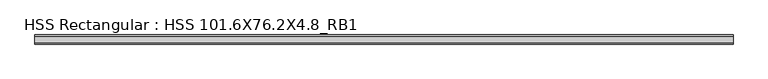
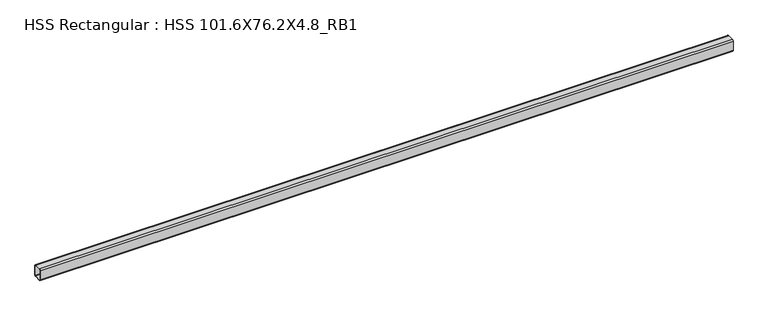
"""IFC4 building model written with IfcOpenShell, lengths in millimetres: beam geometry, HSS Rectangular : HSS 101.6X76.2X4.8_RB1."""

import ifcopenshell
import ifcopenshell.guid

model = None  # the IFC model being written
_history = None  # IfcOwnerHistory: only IFC2X3 demands one
_inside = {}  # id of a spatial element -> (the spatial element, [elements in it])
_under = {}  # id of a project, library or spatial element -> (it, [spatial elements below it])
_declared = {}  # id of a project -> (the project, [libraries it declares])
_typed = {}  # id of a type object -> (the type object, [elements of that type])
_made_of = {}  # id of a material, layer set ... -> (it, [elements and type objects made of it])


def new_model(schema):
    """Start an empty IFC model of exactly this schema.

    Asked for "IFC4X3", IfcOpenShell would pick the latest addendum, in which some entities
    have other attributes; the version numbers below select the first issue.
    IFC2X3 requires an IfcOwnerHistory on every rooted entity: one is made here for all.
    """
    global model, _history
    if schema == "IFC4X3":
        model = ifcopenshell.file(schema_version=(4, 3, 0, 0))
    else:
        model = ifcopenshell.file(schema=schema)
    _inside.clear()
    _under.clear()
    _declared.clear()
    _typed.clear()
    _made_of.clear()
    _history = None
    if model.schema == "IFC2X3":
        org = make("IfcOrganization", Name="unknown")
        user = make(
            "IfcPersonAndOrganization",
            ThePerson=make("IfcPerson", FamilyName="unknown"),
            TheOrganization=org,
        )
        app = make(
            "IfcApplication",
            ApplicationDeveloper=org,
            Version="unknown",
            ApplicationFullName="unknown",
            ApplicationIdentifier="unknown",
        )
        _history = make(
            "IfcOwnerHistory",
            OwningUser=user,
            OwningApplication=app,
            ChangeAction="ADDED",
            CreationDate=0,
        )
    return model


def make(cls, **values):
    """One entity of the class cls with the attributes given. An attribute that is None is left unset."""
    return model.create_entity(
        cls, **{name: value for name, value in values.items() if value is not None}
    )


def rooted(cls, **values):
    """An entity with a GlobalId (a new one), such as an element, a storey or a relation."""
    return make(cls, GlobalId=ifcopenshell.guid.new(), OwnerHistory=_history, **values)


def si_unit(unit_type, name, prefix=None):
    """IfcSIUnit, for example si_unit("LENGTHUNIT", "METRE", prefix="MILLI")."""
    return make("IfcSIUnit", UnitType=unit_type, Prefix=prefix, Name=name)


def assignment(units):
    """IfcUnitAssignment: the units of a project."""
    return None if units is None else make("IfcUnitAssignment", Units=units)


def point(xyz):
    """IfcCartesianPoint."""
    return None if xyz is None else make("IfcCartesianPoint", Coordinates=xyz)


def direction(xyz):
    """IfcDirection."""
    return None if xyz is None else make("IfcDirection", DirectionRatios=xyz)


def frame(location, z_axis=None, x_axis=None):
    """IfcAxis2Placement3D, a coordinate frame: its origin and axes. An axis left out is left unset."""
    return make(
        "IfcAxis2Placement3D",
        Location=point(location),
        Axis=direction(z_axis),
        RefDirection=direction(x_axis),
    )


def frame_2d(location, x_axis=None):
    """IfcAxis2Placement2D, a coordinate frame in the plane: its origin and x axis."""
    return make(
        "IfcAxis2Placement2D", Location=point(location), RefDirection=direction(x_axis)
    )


def origin():
    """The frame at (0, 0, 0) with its axes left unset."""
    return frame((0.0, 0.0, 0.0))


def place(relative_to, where):
    """IfcLocalPlacement: puts the frame where relative to a parent placement (None: the world)."""
    return make(
        "IfcLocalPlacement", PlacementRelTo=relative_to, RelativePlacement=where
    )


def context(
    kind, dimensions, precision=None, world=None, true_north=None, identifier=None
):
    """IfcGeometricRepresentationContext, for example the 3D "Model" context."""
    return make(
        "IfcGeometricRepresentationContext",
        ContextIdentifier=identifier,
        ContextType=kind,
        CoordinateSpaceDimension=dimensions,
        Precision=precision,
        WorldCoordinateSystem=world,
        TrueNorth=true_north,
    )


def project(units=None, contexts=None):
    """IfcProject with its units and contexts."""
    return rooted(
        "IfcProject",
        Name="project",
        RepresentationContexts=contexts,
        UnitsInContext=assignment(units),
    )


def spatial(cls, under=None, at=None, **own):
    """A site, building, storey or space (cls), placed at a placement, below another one or the project."""
    s = rooted(cls, ObjectPlacement=at, **own)
    if under is not None:
        _under.setdefault(under.id(), (under, []))[1].append(s)
    return s


def polyline(points):
    """IfcPolyline through the points."""
    return make("IfcPolyline", Points=[point(p) for p in points])


def circle_curve(where, radius):
    """IfcCircle in the frame where."""
    return make("IfcCircle", Position=where, Radius=radius)


def trimmed(basis, trim1, trim2, sense, master):
    """IfcTrimmedCurve: the piece of a basis curve between two trims."""
    return make(
        "IfcTrimmedCurve",
        BasisCurve=basis,
        Trim1=trim1,
        Trim2=trim2,
        SenseAgreement=sense,
        MasterRepresentation=master,
    )


def segment(curve, same_sense, transition):
    """IfcCompositeCurveSegment."""
    return make(
        "IfcCompositeCurveSegment",
        Transition=transition,
        SameSense=same_sense,
        ParentCurve=curve,
    )


def composite_curve(segments, self_intersect=None):
    """IfcCompositeCurve: segments joined end to end."""
    return make("IfcCompositeCurve", Segments=segments, SelfIntersect=self_intersect)


def outline(outer, holes=None, kind="AREA"):
    """IfcArbitraryClosedProfileDef: a profile drawn as a closed curve; with holes, ...WithVoids."""
    if holes is None:
        return make("IfcArbitraryClosedProfileDef", ProfileType=kind, OuterCurve=outer)
    return make(
        "IfcArbitraryProfileDefWithVoids",
        ProfileType=kind,
        OuterCurve=outer,
        InnerCurves=holes,
    )


def extrude(swept, where, along, depth):
    """IfcExtrudedAreaSolid: the profile swept, set in the frame where, extruded along a direction by depth."""
    return make(
        "IfcExtrudedAreaSolid",
        SweptArea=swept,
        Position=where,
        ExtrudedDirection=direction(along),
        Depth=depth,
    )


def shape(context_of_items, identifier, shape_type, items):
    """IfcShapeRepresentation: the items that make up one representation, for example the "Body"."""
    return make(
        "IfcShapeRepresentation",
        ContextOfItems=context_of_items,
        RepresentationIdentifier=identifier,
        RepresentationType=shape_type,
        Items=items,
    )


def source(mapping_origin, context_of_items, identifier, shape_type, items):
    """IfcRepresentationMap: a shape defined once, which mapped items show again and again."""
    return make(
        "IfcRepresentationMap",
        MappingOrigin=mapping_origin,
        MappedRepresentation=shape(context_of_items, identifier, shape_type, items),
    )


def transform(
    local_origin,
    x_axis=None,
    y_axis=None,
    z_axis=None,
    scale=None,
    scale2=None,
    scale3=None,
    uniform=True,
):
    """IfcCartesianTransformationOperator3D, or its non-uniform kind. x_axis, y_axis, z_axis: its Axis1, 2, 3."""
    if uniform:
        return make(
            "IfcCartesianTransformationOperator3D",
            Axis1=direction(x_axis),
            Axis2=direction(y_axis),
            LocalOrigin=point(local_origin),
            Scale=scale,
            Axis3=direction(z_axis),
        )
    return make(
        "IfcCartesianTransformationOperator3DnonUniform",
        Axis1=direction(x_axis),
        Axis2=direction(y_axis),
        LocalOrigin=point(local_origin),
        Scale=scale,
        Axis3=direction(z_axis),
        Scale2=scale2,
        Scale3=scale3,
    )


def mapped(mapping_source, mapping_target):
    """IfcMappedItem: shows the shape of a source again, moved by a transform."""
    return make(
        "IfcMappedItem", MappingSource=mapping_source, MappingTarget=mapping_target
    )


def made_of(thing, what):
    """Note that an element or type object is made of a material, layer set ...; save() writes the relation."""
    if what is not None:
        _made_of.setdefault(what.id(), (what, []))[1].append(thing)
    return thing


def element(
    cls,
    number,
    at=None,
    inside=None,
    cuts=None,
    type_object=None,
    material=None,
    context=None,
    identifier="Body",
    shape_type=None,
    held_by="IfcProductDefinitionShape",
    body=None,
    shapes=None,
    **own,
):
    """One element of the class cls, such as IfcWall. Its Tag is "e" and its number.

    at: its placement. inside: the storey or other place that contains it. cuts: it is an
    opening in that element (IfcRelVoidsElement). A single representation is given by context,
    identifier, shape_type and body (its items); several are given by shapes. held_by: the class
    of the entity that holds the representations. save() writes the other relations.
    """
    e = rooted(cls, Tag="e%d" % number, ObjectPlacement=at, **own)
    if body is not None:
        shapes = [shape(context, identifier, shape_type, body)]
    if shapes is not None:
        e.Representation = make(held_by, Representations=shapes)
    if inside is not None:
        _inside.setdefault(inside.id(), (inside, []))[1].append(e)
    if cuts is not None:
        rooted(
            "IfcRelVoidsElement", RelatingBuildingElement=cuts, RelatedOpeningElement=e
        )
    if type_object is not None:
        _typed.setdefault(type_object.id(), (type_object, []))[1].append(e)
    return made_of(e, material)


def aggregate(whole, parts):
    """IfcRelAggregates: a whole, such as a stair, and the parts it consists of."""
    return rooted("IfcRelAggregates", RelatingObject=whole, RelatedObjects=parts)


def save(model, path):
    """Write the relations noted so far, then the file.

    IfcRelAggregates (storeys below a building ...), IfcRelContainedInSpatialStructure (elements
    in a storey), IfcRelDefinesByType, IfcRelAssociatesMaterial and IfcRelDeclares: one each for
    every whole, place, type object, material and project.
    """
    for whole, parts in _under.values():
        aggregate(whole, parts)
    for where, things in _inside.values():
        rooted(
            "IfcRelContainedInSpatialStructure",
            RelatedElements=things,
            RelatingStructure=where,
        )
    for kind, things in _typed.values():
        rooted("IfcRelDefinesByType", RelatedObjects=things, RelatingType=kind)
    for what, things in _made_of.values():
        rooted("IfcRelAssociatesMaterial", RelatedObjects=things, RelatingMaterial=what)
    for by, libraries in _declared.values():
        rooted("IfcRelDeclares", RelatingContext=by, RelatedDefinitions=libraries)
    model.write(path)


def hss_rectangular_hss_101_6x76_2x4_8_rb1_d55246ad(model_context):
    return source(origin(), model_context, "Body", "SweptSolid", [
        extrude(outline(composite_curve([segment(polyline([(38.1, 41.275), (38.1, -41.275)]), True, "CONTINUOUS"), segment(trimmed(circle_curve(frame_2d((28.575, -41.275)), 9.525), [point((38.1, -41.275))], [point((28.575, -50.8))], False, "CARTESIAN"), True, "CONTINUOUS"), segment(polyline([(28.575, -50.8), (-28.575, -50.8)]), True, "CONTINUOUS"), segment(trimmed(circle_curve(frame_2d((-28.575, -41.275)), 9.525), [point((-28.575, -50.8))], [point((-38.1, -41.275))], False, "CARTESIAN"), True, "CONTINUOUS"), segment(polyline([(-38.1, -41.275), (-38.1, 41.275)]), True, "CONTINUOUS"), segment(trimmed(circle_curve(frame_2d((-28.575, 41.275)), 9.525), [point((-38.1, 41.275))], [point((-28.575, 50.8))], False, "CARTESIAN"), True, "CONTINUOUS"), segment(polyline([(-28.575, 50.8), (28.575, 50.8)]), True, "CONTINUOUS"), segment(trimmed(circle_curve(frame_2d((28.575, 41.275)), 9.525), [point((28.575, 50.8))], [point((38.1, 41.275))], False, "CARTESIAN"), True, "CONTINUOUS")], self_intersect=False), holes=[composite_curve([segment(trimmed(circle_curve(frame_2d((-28.575, 41.275)), 4.7625), [point((-28.575, 46.0375))], [point((-33.3375, 41.275))], True, "CARTESIAN"), True, "CONTINUOUS"), segment(polyline([(-33.3375, 41.275), (-33.3375, -41.275)]), True, "CONTINUOUS"), segment(trimmed(circle_curve(frame_2d((-28.575, -41.275)), 4.7625), [point((-33.3375, -41.275))], [point((-28.575, -46.0375))], True, "CARTESIAN"), True, "CONTINUOUS"), segment(polyline([(-28.575, -46.0375), (28.575, -46.0375)]), True, "CONTINUOUS"), segment(trimmed(circle_curve(frame_2d((28.575, -41.275)), 4.7625), [point((28.575, -46.0375))], [point((33.3375, -41.275))], True, "CARTESIAN"), True, "CONTINUOUS"), segment(polyline([(33.3375, -41.275), (33.3375, 41.275)]), True, "CONTINUOUS"), segment(trimmed(circle_curve(frame_2d((28.575, 41.275)), 4.7625), [point((33.3375, 41.275))], [point((28.575, 46.0375))], True, "CARTESIAN"), True, "CONTINUOUS"), segment(polyline([(28.575, 46.0375), (-28.575, 46.0375)]), True, "CONTINUOUS")], self_intersect=False)]), frame((-7467.2727012, 0.0, 0.0), z_axis=(1.0, 0.0, 0.0), x_axis=(0.0, 1.0, 0.0)), (0.0, 0.0, 1.0), 5840.0992104),
    ])


if __name__ == "__main__":
    model = new_model("IFC4")
    model_context = context("Model", 3, world=origin())
    ifc_project = project(units=[si_unit("LENGTHUNIT", "METRE", prefix="MILLI")], contexts=[model_context])
    site = spatial("IfcSite", under=ifc_project)
    building = spatial("IfcBuilding", under=site)
    placement = place(None, origin())
    hss_rectangular_hss_101_6x76_2x4_8_rb1_shape = hss_rectangular_hss_101_6x76_2x4_8_rb1_d55246ad(model_context)
    element("IfcBeam", 1, ObjectType="HSS Rectangular : HSS 101.6X76.2X4.8_RB1", at=placement, inside=building, context=model_context, shape_type="MappedRepresentation", body=[
        mapped(hss_rectangular_hss_101_6x76_2x4_8_rb1_shape, transform((0.0, 0.0, 0.0), x_axis=(1.0, 0.0, 0.0), y_axis=(0.0, 1.0, 0.0), z_axis=(0.0, 0.0, 1.0))),
    ])
    save(model, "model.ifc")

# Revit data of these elements
# Type "HSS Rectangular : HSS 101.6X76.2X4.8_RB1"
#   Section Name Key = "HSS 4X3X3/16"
#   Assembly Code = "B10"
#   Width = 7.62 cm
#   Wall Nominal Thickness = 0.4763 cm
#   Wall Design Thickness = 0.442 cm
#   Torsional Moment of Inertia = 260.561 cm⁴
#   Torsional Modulus = 61.2876 cm³
#   Section Area = 14.4516 cm²
#   Plastic Modulus weak axis = 40.3122 cm³
#   Plastic Modulus strong axis = 49.1612 cm³
#   Perimeter = 0.881482 m²/m
#   Outer Fillet = 0.9525 cm
#   Nominal Weight = 12.1285 kgf/m
#   Moment of Inertia weak axis = 131.529 cm⁴
#   Moment of Inertia strong axis = 205.202 cm⁴
#   Inner Fillet = 0.4763 cm
#   Height = 10.16 cm
#   Elastic Modulus weak axis = 34.4128 cm³
#   Elastic Modulus strong axis = 40.476 cm³
#   Centroid Vertical = 5.08 cm
#   Centroid Horizontal = 3.81 cm
#   Length [instance default] = 1524 mm
#   Structural Material [instance default] = Steel ASTM A500, Grade B, Rectangular and Square
#   Principal Axes Angle = 0
# Element 1 (IfcBeam, "HSS Rectangular : HSS 101.6X76.2X4.8_RB1")
#   Structural Material = Steel ASTM A992
#   Materials on its faces: "Steel ASTM A992"
# Materials
#   "Steel ASTM A500, Grade B, Rectangular and Square": class "Metal", colour RGB 199 199 199, transparency 0, Description = "Carbon steel", Cost = 0
#   "Steel ASTM A992": class "Metal", colour RGB 199 199 199, transparency 0, Description = "Structural steel 50ksi", Cost = 0
